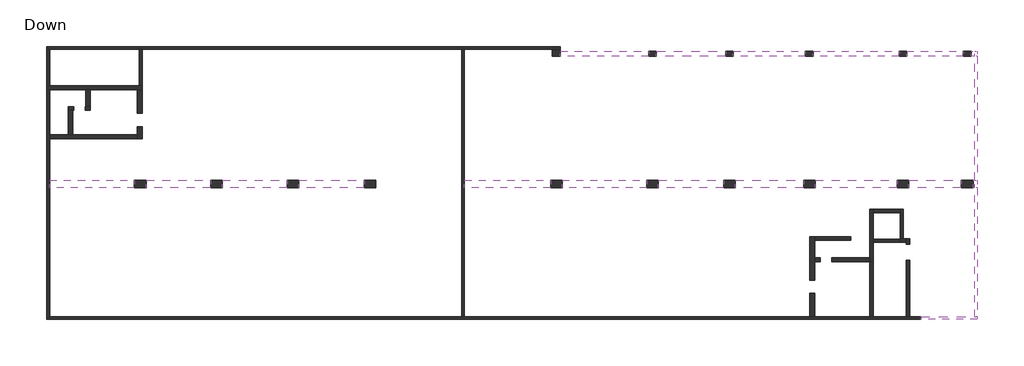
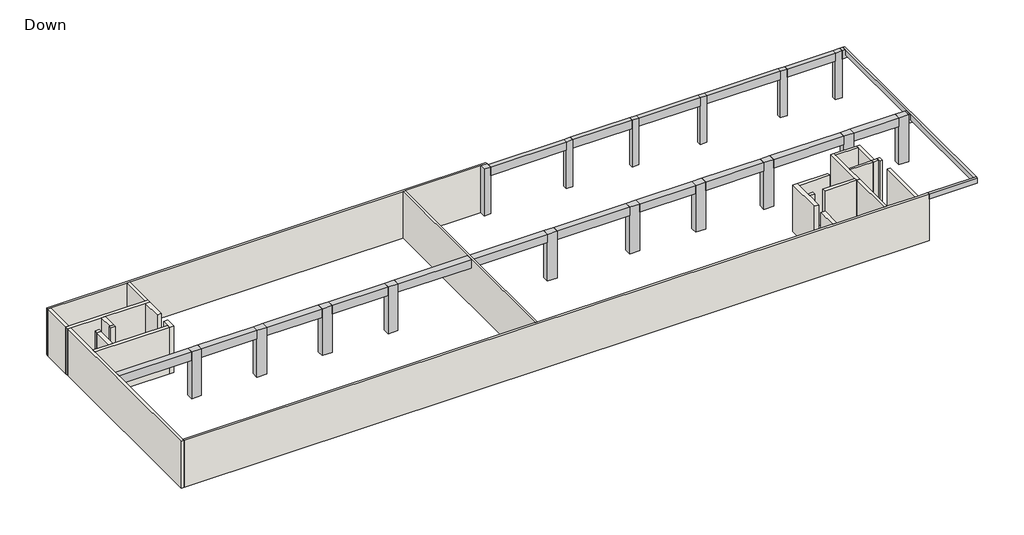
# One storey: 27 walls, 19 beams, 16 columns.
# Revit data of these elements (continued)
# Element 37 (IfcWall, "20") (continued)
#   Materials on its faces: "Concrete"
# Element 38 (IfcWall, "20")
#   Comments = ""
#   Mark = "W3"
#   SOFiSTiK_AMG_Comments = ""
#   Top Offset = 0 cm
#   Base Offset = 0 cm
#   wall height = 450 cm
#   SOFiSTiK_AMG_Scheduled = yes
#   SOFiSTiK_AMG_Adjusted = yes
#   Phase Created = New Construction
#   Base Constraint = Down
#   Top Constraint = Typical Floor
#   Materials on its faces: "Concrete"
# Element 39 (IfcWall, "20")
#   Comments = ""
#   Mark = "W4"
#   SOFiSTiK_AMG_Comments = ""
#   Top Offset = 0 cm
#   Base Offset = 0 cm
#   wall height = 450 cm
#   SOFiSTiK_AMG_Scheduled = yes
#   SOFiSTiK_AMG_Adjusted = yes
#   Phase Created = New Construction
#   Base Constraint = Down
#   Top Constraint = Typical Floor
#   Materials on its faces: "Concrete"
# Element 40 (IfcWall, "23")
#   Comments = ""
#   Mark = "W5"
#   SOFiSTiK_AMG_Comments = ""
#   Top Offset = 0 cm
#   Base Offset = 0 cm
#   wall height = 450 cm
#   SOFiSTiK_AMG_Scheduled = yes
#   SOFiSTiK_AMG_Adjusted = yes
#   Phase Created = New Construction
#   Base Constraint = Down
#   Top Constraint = Typical Floor
#   Materials on its faces: "Concrete"
# Element 41 (IfcWall, "25")
#   Comments = ""
#   Mark = "W11"
#   SOFiSTiK_AMG_Comments = ""
#   Top Offset = 0 cm
#   Base Offset = 0 cm
#   wall height = 450 cm
#   SOFiSTiK_AMG_Scheduled = yes
#   SOFiSTiK_AMG_Adjusted = yes
#   Phase Created = New Construction
#   Base Constraint = Down
#   Top Constraint = Typical Floor
#   Materials on its faces: "Concrete"
# Element 42 (IfcWall, "25")
#   Comments = ""
#   Mark = "W12"
#   SOFiSTiK_AMG_Comments = ""
#   Top Offset = 0 cm
#   Base Offset = 0 cm
#   wall height = 450 cm
#   SOFiSTiK_AMG_Scheduled = yes
#   SOFiSTiK_AMG_Adjusted = yes
#   Phase Created = New Construction
#   Base Constraint = Down
#   Top Constraint = Typical Floor
#   Materials on its faces: "Concrete"
# Element 43 (IfcWall, "25")
#   Comments = ""
#   Mark = "W13"
#   SOFiSTiK_AMG_Comments = ""
#   Top Offset = 0 cm
#   Base Offset = 0 cm
#   wall height = 450 cm
#   SOFiSTiK_AMG_Scheduled = yes
#   SOFiSTiK_AMG_Adjusted = yes
#   Phase Created = New Construction
#   Base Constraint = Down
#   Top Constraint = Typical Floor
#   Materials on its faces: "Concrete"
# Element 44 (IfcWall, "25")
#   Comments = ""
#   Mark = "W14"
#   SOFiSTiK_AMG_Comments = ""
#   Top Offset = 0 cm
#   Base Offset = 0 cm
#   wall height = 450 cm
#   SOFiSTiK_AMG_Scheduled = yes
#   SOFiSTiK_AMG_Adjusted = yes
#   Phase Created = New Construction
#   Base Constraint = Down
#   Top Constraint = Typical Floor
#   Materials on its faces: "Concrete"
# Element 45 (IfcWall, "25")
#   Comments = ""
#   Mark = "W15"
#   SOFiSTiK_AMG_Comments = ""
#   Top Offset = 0 cm
#   Base Offset = 0 cm
#   wall height = 450 cm
#   SOFiSTiK_AMG_Scheduled = yes
#   SOFiSTiK_AMG_Adjusted = yes
#   Phase Created = New Construction
#   Base Constraint = Down
#   Top Constraint = Typical Floor
#   Materials on its faces: "Concrete"
# Element 46 (IfcWall, "25")
#   Comments = ""
#   Mark = "W16"
#   SOFiSTiK_AMG_Comments = ""
#   Top Offset = 0 cm
#   Base Offset = 0 cm
#   wall height = 450 cm
#   SOFiSTiK_AMG_Scheduled = yes
#   SOFiSTiK_AMG_Adjusted = yes
#   Phase Created = New Construction
#   Base Constraint = Down
#   Top Constraint = Typical Floor
#   Materials on its faces: "Concrete"
# Element 47 (IfcWall, "25")
#   Comments = ""
#   Mark = "W17"
#   SOFiSTiK_AMG_Comments = ""
#   Top Offset = 0 cm
#   Base Offset = 0 cm
#   wall height = 450 cm
#   SOFiSTiK_AMG_Scheduled = yes
#   SOFiSTiK_AMG_Adjusted = yes
#   Phase Created = New Construction
#   Base Constraint = Down
#   Top Constraint = Typical Floor
#   Materials on its faces: "Concrete"
# Element 48 (IfcWall, "25")
#   Comments = ""
#   Mark = "W18"
#   SOFiSTiK_AMG_Comments = ""
#   Top Offset = 0 cm
#   Base Offset = 0 cm
#   wall height = 450 cm
#   SOFiSTiK_AMG_Scheduled = yes
#   SOFiSTiK_AMG_Adjusted = yes
#   Phase Created = New Construction
#   Base Constraint = Down
#   Top Constraint = Typical Floor
#   Materials on its faces: "Concrete"
# Element 49 (IfcWall, "27")
#   Comments = ""
#   Mark = "W19"
#   SOFiSTiK_AMG_Comments = ""
#   Top Offset = 0 cm
#   Base Offset = 0 cm
#   wall height = 450 cm
#   SOFiSTiK_AMG_Scheduled = yes
#   SOFiSTiK_AMG_Adjusted = yes
#   Phase Created = New Construction
#   Base Constraint = Down
#   Top Constraint = Typical Floor
#   Materials on its faces: "Concrete"
# Element 50 (IfcWall, "27")
#   Comments = ""
#   Mark = "W20"
#   SOFiSTiK_AMG_Comments = ""
#   Top Offset = 0 cm
#   Base Offset = 0 cm
#   wall height = 450 cm
#   SOFiSTiK_AMG_Scheduled = yes
#   SOFiSTiK_AMG_Adjusted = yes
#   Phase Created = New Construction
#   Base Constraint = Down
#   Top Constraint = Typical Floor
#   Materials on its faces: "Concrete"
# Element 51 (IfcWall, "27")
#   Comments = ""
#   Mark = "W21"
#   SOFiSTiK_AMG_Comments = ""
#   Top Offset = 0 cm
#   Base Offset = 0 cm
#   wall height = 450 cm
#   SOFiSTiK_AMG_Scheduled = yes
#   SOFiSTiK_AMG_Adjusted = yes
#   Phase Created = New Construction
#   Base Constraint = Down
#   Top Constraint = Typical Floor
#   Materials on its faces: "Concrete"
# Element 52 (IfcWall, "30")
#   Comments = ""
#   Mark = "W6"
#   SOFiSTiK_AMG_Comments = ""
#   Top Offset = 0 cm
#   Base Offset = 0 cm
#   wall height = 450 cm
#   SOFiSTiK_AMG_Scheduled = yes
#   SOFiSTiK_AMG_Adjusted = yes
#   Phase Created = New Construction
#   Base Constraint = Down
#   Top Constraint = Typical Floor
#   Materials on its faces: "Concrete"
# Element 53 (IfcWall, "30")
#   Comments = ""
#   Mark = "W7"
#   SOFiSTiK_AMG_Comments = ""
#   Top Offset = 0 cm
#   Base Offset = 0 cm
#   wall height = 450 cm
#   SOFiSTiK_AMG_Scheduled = yes
#   SOFiSTiK_AMG_Adjusted = yes
#   Phase Created = New Construction
#   Base Constraint = Down
#   Top Constraint = Typical Floor
#   Materials on its faces: "Concrete"
# Element 54 (IfcWall, "30")
#   Comments = ""
#   Mark = "W8"
#   SOFiSTiK_AMG_Comments = ""
#   Top Offset = 0 cm
#   Base Offset = 0 cm
#   wall height = 450 cm
#   SOFiSTiK_AMG_Scheduled = yes
#   SOFiSTiK_AMG_Adjusted = yes
#   Phase Created = New Construction
#   Base Constraint = Down
#   Top Constraint = Typical Floor
#   Materials on its faces: "Concrete"
# Element 55 (IfcWall, "30")
#   Comments = ""
#   Mark = "W9"
#   SOFiSTiK_AMG_Comments = ""
#   Top Offset = 0 cm
#   Base Offset = 0 cm
#   wall height = 450 cm
#   SOFiSTiK_AMG_Scheduled = yes
#   SOFiSTiK_AMG_Adjusted = yes
#   Phase Created = New Construction
#   Base Constraint = Down
#   Top Constraint = Typical Floor
#   Materials on its faces: "Concrete"
# Element 56 (IfcWall, "30")
#   Comments = ""
#   Mark = "W10"
#   SOFiSTiK_AMG_Comments = ""
#   Top Offset = 0 cm
#   Base Offset = 0 cm
#   wall height = 450 cm
#   SOFiSTiK_AMG_Scheduled = yes
#   SOFiSTiK_AMG_Adjusted = yes
#   Phase Created = New Construction
#   Base Constraint = Down
#   Top Constraint = Typical Floor
#   Materials on its faces: "Concrete"
# Element 57 (IfcWall, "35")
#   Comments = ""
#   Mark = "W26"
#   SOFiSTiK_AMG_Comments = ""
#   Top Offset = 0 cm
#   Base Offset = 0 cm
#   wall height = 450 cm
#   SOFiSTiK_AMG_Scheduled = yes
#   SOFiSTiK_AMG_Adjusted = yes
#   Phase Created = New Construction
#   Base Constraint = Down
#   Top Constraint = Typical Floor
#   Materials on its faces: "Concrete"
# Element 58 (IfcWall, "35")
#   Comments = ""
#   Mark = "W27"
#   SOFiSTiK_AMG_Comments = ""
#   Top Offset = 0 cm
#   Base Offset = 0 cm
#   wall height = 450 cm
#   SOFiSTiK_AMG_Scheduled = yes
#   SOFiSTiK_AMG_Adjusted = yes
#   Phase Created = New Construction
#   Base Constraint = Down
#   Top Constraint = Typical Floor
#   Materials on its faces: "Concrete"
# Element 59 (IfcWall, "40")
#   Comments = ""
#   Mark = "W22"
#   SOFiSTiK_AMG_Comments = ""
#   Top Offset = 0 cm
#   Base Offset = 0 cm
#   wall height = 450 cm
#   SOFiSTiK_AMG_Scheduled = yes
#   SOFiSTiK_AMG_Adjusted = yes
#   Phase Created = New Construction
#   Base Constraint = Down
#   Top Constraint = Typical Floor
#   Materials on its faces: "Concrete"
# Element 60 (IfcWall, "40")
#   Comments = ""
#   Mark = "W23"
#   SOFiSTiK_AMG_Comments = ""
#   Top Offset = 0 cm
#   Base Offset = 0 cm
#   wall height = 450 cm
#   SOFiSTiK_AMG_Scheduled = yes
#   SOFiSTiK_AMG_Adjusted = yes
#   Phase Created = New Construction
#   Base Constraint = Down
#   Top Constraint = Typical Floor
#   Materials on its faces: "Concrete"
# Element 61 (IfcWall, "40")
#   Comments = ""
#   Mark = "W24"
#   SOFiSTiK_AMG_Comments = ""
#   Top Offset = 0 cm
#   Base Offset = 0 cm
#   wall height = 450 cm
#   SOFiSTiK_AMG_Scheduled = yes
#   SOFiSTiK_AMG_Adjusted = yes
#   Phase Created = New Construction
#   Base Constraint = Down
#   Top Constraint = Typical Floor
#   Materials on its faces: "Concrete"
# Element 62 (IfcWall, "40")
#   Comments = ""
#   Mark = "W25"
#   SOFiSTiK_AMG_Comments = ""
#   Top Offset = 0 cm
#   Base Offset = 0 cm
#   wall height = 450 cm
#   SOFiSTiK_AMG_Scheduled = yes
#   SOFiSTiK_AMG_Adjusted = yes
#   Phase Created = New Construction
#   Base Constraint = Down
#   Top Constraint = Typical Floor
#   Materials on its faces: "Concrete"
# Materials
#   "Concrete": class "Concrete", colour RGB 192 192 192, transparency 0, Keynote = "01000", Description = "Cast-in-place concrete", Cost = 0
